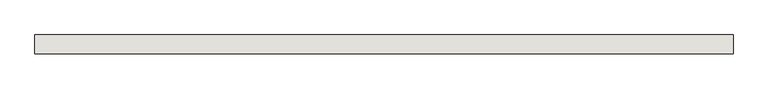
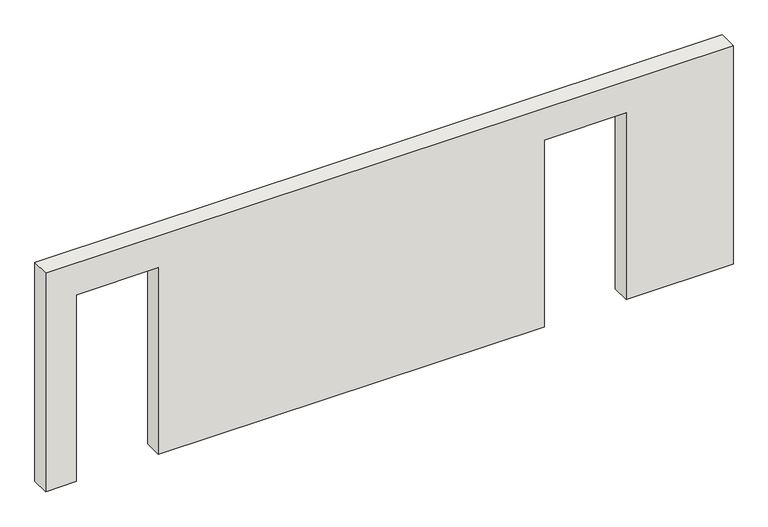
"""IFC4 building model written with IfcOpenShell, lengths in millimetres: wall geometry, Holzwand."""

from ifc_helpers import new_model, si_unit, frame, origin, place, context, project, spatial, polyline, outline, extrude, source, transform, mapped, element, save


def wall_13859d00(model_context):
    return source(origin(), model_context, "Body", "SweptSolid", [
        extrude(outline(polyline([(0.0, 331.2957264), (2135.0, 331.2957264), (2135.0, 1216.2957264), (0.0, 1216.2957264), (0.0, 5383.8534032), (2135.0, 5383.8534032), (2135.0, 6268.8534032), (0.0, 6268.8534032), (0.0, 7425.0), (2500.0, 7425.0), (2500.0, 0.0), (0.0, 0.0), (0.0, 331.2957264)])), frame((0.0, 0.0, 0.0), z_axis=(0.0, 1.0, 0.0), x_axis=(0.0, 0.0, 1.0)), (0.0, 0.0, 1.0), 200.0),
    ])


if __name__ == "__main__":
    model = new_model("IFC4")
    model_context = context("Model", 3, world=origin())
    ifc_project = project(units=[si_unit("LENGTHUNIT", "METRE", prefix="MILLI")], contexts=[model_context])
    site = spatial("IfcSite", under=ifc_project)
    building = spatial("IfcBuilding", under=site)
    placement = place(None, origin())
    wall_shape = wall_13859d00(model_context)
    element("IfcWall", 1, ObjectType="Holzwand", at=placement, inside=building, context=model_context, shape_type="MappedRepresentation", body=[
        mapped(wall_shape, transform((0.0, 0.0, 0.0), x_axis=(1.0, 0.0, 0.0), y_axis=(0.0, 1.0, 0.0), z_axis=(0.0, 0.0, 1.0))),
    ])
    save(model, "model.ifc")

# Revit data of these elements
# Element 1 (IfcWall, "Holzwand")
#   Materials on its faces: "holzschalung"
# Materials
#   "holzschalung": class "Unassigned", colour RGB 128 128 128, transparency 0
